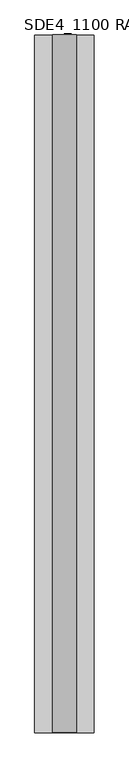
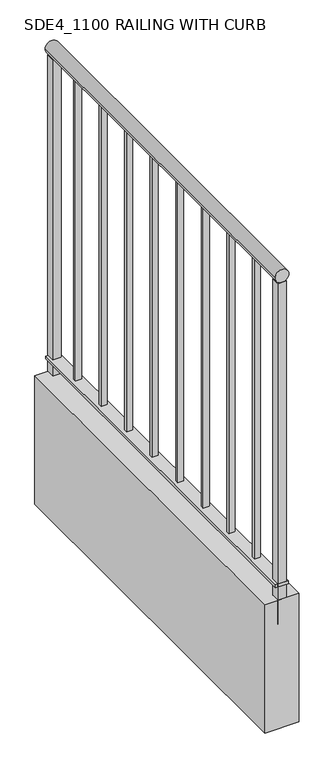
"""IFC4 building model written with IfcOpenShell, lengths in millimetres: railing geometry, SDE4_1100 RAILING WITH CURB."""

import ifcopenshell
import ifcopenshell.guid

model = None  # the IFC model being written
_history = None  # IfcOwnerHistory: only IFC2X3 demands one
_inside = {}  # id of a spatial element -> (the spatial element, [elements in it])
_under = {}  # id of a project, library or spatial element -> (it, [spatial elements below it])
_declared = {}  # id of a project -> (the project, [libraries it declares])
_typed = {}  # id of a type object -> (the type object, [elements of that type])
_made_of = {}  # id of a material, layer set ... -> (it, [elements and type objects made of it])


def new_model(schema):
    """Start an empty IFC model of exactly this schema.

    Asked for "IFC4X3", IfcOpenShell would pick the latest addendum, in which some entities
    have other attributes; the version numbers below select the first issue.
    IFC2X3 requires an IfcOwnerHistory on every rooted entity: one is made here for all.
    """
    global model, _history
    if schema == "IFC4X3":
        model = ifcopenshell.file(schema_version=(4, 3, 0, 0))
    else:
        model = ifcopenshell.file(schema=schema)
    _inside.clear()
    _under.clear()
    _declared.clear()
    _typed.clear()
    _made_of.clear()
    _history = None
    if model.schema == "IFC2X3":
        org = make("IfcOrganization", Name="unknown")
        user = make(
            "IfcPersonAndOrganization",
            ThePerson=make("IfcPerson", FamilyName="unknown"),
            TheOrganization=org,
        )
        app = make(
            "IfcApplication",
            ApplicationDeveloper=org,
            Version="unknown",
            ApplicationFullName="unknown",
            ApplicationIdentifier="unknown",
        )
        _history = make(
            "IfcOwnerHistory",
            OwningUser=user,
            OwningApplication=app,
            ChangeAction="ADDED",
            CreationDate=0,
        )
    return model


def make(cls, **values):
    """One entity of the class cls with the attributes given. An attribute that is None is left unset."""
    return model.create_entity(
        cls, **{name: value for name, value in values.items() if value is not None}
    )


def rooted(cls, **values):
    """An entity with a GlobalId (a new one), such as an element, a storey or a relation."""
    return make(cls, GlobalId=ifcopenshell.guid.new(), OwnerHistory=_history, **values)


def si_unit(unit_type, name, prefix=None):
    """IfcSIUnit, for example si_unit("LENGTHUNIT", "METRE", prefix="MILLI")."""
    return make("IfcSIUnit", UnitType=unit_type, Prefix=prefix, Name=name)


def assignment(units):
    """IfcUnitAssignment: the units of a project."""
    return None if units is None else make("IfcUnitAssignment", Units=units)


def point(xyz):
    """IfcCartesianPoint."""
    return None if xyz is None else make("IfcCartesianPoint", Coordinates=xyz)


def direction(xyz):
    """IfcDirection."""
    return None if xyz is None else make("IfcDirection", DirectionRatios=xyz)


def frame(location, z_axis=None, x_axis=None):
    """IfcAxis2Placement3D, a coordinate frame: its origin and axes. An axis left out is left unset."""
    return make(
        "IfcAxis2Placement3D",
        Location=point(location),
        Axis=direction(z_axis),
        RefDirection=direction(x_axis),
    )


def frame_2d(location, x_axis=None):
    """IfcAxis2Placement2D, a coordinate frame in the plane: its origin and x axis."""
    return make(
        "IfcAxis2Placement2D", Location=point(location), RefDirection=direction(x_axis)
    )


def origin():
    """The frame at (0, 0, 0) with its axes left unset."""
    return frame((0.0, 0.0, 0.0))


def place(relative_to, where):
    """IfcLocalPlacement: puts the frame where relative to a parent placement (None: the world)."""
    return make(
        "IfcLocalPlacement", PlacementRelTo=relative_to, RelativePlacement=where
    )


def context(
    kind, dimensions, precision=None, world=None, true_north=None, identifier=None
):
    """IfcGeometricRepresentationContext, for example the 3D "Model" context."""
    return make(
        "IfcGeometricRepresentationContext",
        ContextIdentifier=identifier,
        ContextType=kind,
        CoordinateSpaceDimension=dimensions,
        Precision=precision,
        WorldCoordinateSystem=world,
        TrueNorth=true_north,
    )


def project(units=None, contexts=None):
    """IfcProject with its units and contexts."""
    return rooted(
        "IfcProject",
        Name="project",
        RepresentationContexts=contexts,
        UnitsInContext=assignment(units),
    )


def spatial(cls, under=None, at=None, **own):
    """A site, building, storey or space (cls), placed at a placement, below another one or the project."""
    s = rooted(cls, ObjectPlacement=at, **own)
    if under is not None:
        _under.setdefault(under.id(), (under, []))[1].append(s)
    return s


def polyline(points):
    """IfcPolyline through the points."""
    return make("IfcPolyline", Points=[point(p) for p in points])


def circle_curve(where, radius):
    """IfcCircle in the frame where."""
    return make("IfcCircle", Position=where, Radius=radius)


def trimmed(basis, trim1, trim2, sense, master):
    """IfcTrimmedCurve: the piece of a basis curve between two trims."""
    return make(
        "IfcTrimmedCurve",
        BasisCurve=basis,
        Trim1=trim1,
        Trim2=trim2,
        SenseAgreement=sense,
        MasterRepresentation=master,
    )


def segment(curve, same_sense, transition):
    """IfcCompositeCurveSegment."""
    return make(
        "IfcCompositeCurveSegment",
        Transition=transition,
        SameSense=same_sense,
        ParentCurve=curve,
    )


def composite_curve(segments, self_intersect=None):
    """IfcCompositeCurve: segments joined end to end."""
    return make("IfcCompositeCurve", Segments=segments, SelfIntersect=self_intersect)


def outline(outer, holes=None, kind="AREA"):
    """IfcArbitraryClosedProfileDef: a profile drawn as a closed curve; with holes, ...WithVoids."""
    if holes is None:
        return make("IfcArbitraryClosedProfileDef", ProfileType=kind, OuterCurve=outer)
    return make(
        "IfcArbitraryProfileDefWithVoids",
        ProfileType=kind,
        OuterCurve=outer,
        InnerCurves=holes,
    )


def extrude(swept, where, along, depth):
    """IfcExtrudedAreaSolid: the profile swept, set in the frame where, extruded along a direction by depth."""
    return make(
        "IfcExtrudedAreaSolid",
        SweptArea=swept,
        Position=where,
        ExtrudedDirection=direction(along),
        Depth=depth,
    )


def shape(context_of_items, identifier, shape_type, items):
    """IfcShapeRepresentation: the items that make up one representation, for example the "Body"."""
    return make(
        "IfcShapeRepresentation",
        ContextOfItems=context_of_items,
        RepresentationIdentifier=identifier,
        RepresentationType=shape_type,
        Items=items,
    )


def source(mapping_origin, context_of_items, identifier, shape_type, items):
    """IfcRepresentationMap: a shape defined once, which mapped items show again and again."""
    return make(
        "IfcRepresentationMap",
        MappingOrigin=mapping_origin,
        MappedRepresentation=shape(context_of_items, identifier, shape_type, items),
    )


def transform(
    local_origin,
    x_axis=None,
    y_axis=None,
    z_axis=None,
    scale=None,
    scale2=None,
    scale3=None,
    uniform=True,
):
    """IfcCartesianTransformationOperator3D, or its non-uniform kind. x_axis, y_axis, z_axis: its Axis1, 2, 3."""
    if uniform:
        return make(
            "IfcCartesianTransformationOperator3D",
            Axis1=direction(x_axis),
            Axis2=direction(y_axis),
            LocalOrigin=point(local_origin),
            Scale=scale,
            Axis3=direction(z_axis),
        )
    return make(
        "IfcCartesianTransformationOperator3DnonUniform",
        Axis1=direction(x_axis),
        Axis2=direction(y_axis),
        LocalOrigin=point(local_origin),
        Scale=scale,
        Axis3=direction(z_axis),
        Scale2=scale2,
        Scale3=scale3,
    )


def mapped(mapping_source, mapping_target):
    """IfcMappedItem: shows the shape of a source again, moved by a transform."""
    return make(
        "IfcMappedItem", MappingSource=mapping_source, MappingTarget=mapping_target
    )


def made_of(thing, what):
    """Note that an element or type object is made of a material, layer set ...; save() writes the relation."""
    if what is not None:
        _made_of.setdefault(what.id(), (what, []))[1].append(thing)
    return thing


def element(
    cls,
    number,
    at=None,
    inside=None,
    cuts=None,
    type_object=None,
    material=None,
    context=None,
    identifier="Body",
    shape_type=None,
    held_by="IfcProductDefinitionShape",
    body=None,
    shapes=None,
    **own,
):
    """One element of the class cls, such as IfcWall. Its Tag is "e" and its number.

    at: its placement. inside: the storey or other place that contains it. cuts: it is an
    opening in that element (IfcRelVoidsElement). A single representation is given by context,
    identifier, shape_type and body (its items); several are given by shapes. held_by: the class
    of the entity that holds the representations. save() writes the other relations.
    """
    e = rooted(cls, Tag="e%d" % number, ObjectPlacement=at, **own)
    if body is not None:
        shapes = [shape(context, identifier, shape_type, body)]
    if shapes is not None:
        e.Representation = make(held_by, Representations=shapes)
    if inside is not None:
        _inside.setdefault(inside.id(), (inside, []))[1].append(e)
    if cuts is not None:
        rooted(
            "IfcRelVoidsElement", RelatingBuildingElement=cuts, RelatedOpeningElement=e
        )
    if type_object is not None:
        _typed.setdefault(type_object.id(), (type_object, []))[1].append(e)
    return made_of(e, material)


def aggregate(whole, parts):
    """IfcRelAggregates: a whole, such as a stair, and the parts it consists of."""
    return rooted("IfcRelAggregates", RelatingObject=whole, RelatedObjects=parts)


def save(model, path):
    """Write the relations noted so far, then the file.

    IfcRelAggregates (storeys below a building ...), IfcRelContainedInSpatialStructure (elements
    in a storey), IfcRelDefinesByType, IfcRelAssociatesMaterial and IfcRelDeclares: one each for
    every whole, place, type object, material and project.
    """
    for whole, parts in _under.values():
        aggregate(whole, parts)
    for where, things in _inside.values():
        rooted(
            "IfcRelContainedInSpatialStructure",
            RelatedElements=things,
            RelatingStructure=where,
        )
    for kind, things in _typed.values():
        rooted("IfcRelDefinesByType", RelatedObjects=things, RelatingType=kind)
    for what, things in _made_of.values():
        rooted("IfcRelAssociatesMaterial", RelatedObjects=things, RelatingMaterial=what)
    for by, libraries in _declared.values():
        rooted("IfcRelDeclares", RelatingContext=by, RelatedDefinitions=libraries)
    model.write(path)


def sde4_1100_railing_with_curb_01aa2083(model_context):
    return source(origin(), model_context, "Body", "SweptSolid", [
        extrude(outline(composite_curve([segment(trimmed(circle_curve(frame_2d((131550.0, 76500.4)), 20.0), [point((131550.0, 76520.4))], [point((131550.0, 76480.4))], False, "CARTESIAN"), True, "CONTINUOUS"), segment(trimmed(circle_curve(frame_2d((131550.0, 76500.4)), 20.0), [point((131550.0, 76480.4))], [point((131550.0, 76520.4))], False, "CARTESIAN"), True, "CONTINUOUS")], self_intersect=False)), frame((0.0, 20915.0, 0.0), z_axis=(0.0, 1.0, 0.0), x_axis=(0.0, 0.0, 1.0)), (0.0, 0.0, 1.0), 1174.1666667),
        extrude(outline(polyline([(76481.4, 22089.1666667), (76519.4, 22089.1666667), (76519.4, 20915.0), (76481.4, 20915.0), (76481.4, 22089.1666667)])), frame((0.0, 0.0, 130586.0), z_axis=(0.0, 0.0, 1.0), x_axis=(1.0, 0.0, 0.0)), (0.0, 0.0, 1.0), 9.0),
        extrude(outline(polyline([(76450.0, 22089.1666667), (76550.0, 22089.1666667), (76550.0, 20915.0), (76450.0, 20915.0), (76450.0, 22089.1666667)])), frame((0.0, 0.0, 130145.0), z_axis=(0.0, 0.0, 1.0), x_axis=(1.0, 0.0, 0.0)), (0.0, 0.0, 1.0), 400.0),
        extrude(outline(polyline([(76491.4, 21049.962963), (76509.4, 21049.962963), (76509.4, 21040.962963), (76491.4, 21040.962963), (76491.4, 21049.962963)])), frame((0.0, 0.0, 130595.0), z_axis=(0.0, 0.0, 1.0), x_axis=(1.0, 0.0, 0.0)), (0.0, 0.0, 1.0), 935.0),
        extrude(outline(polyline([(76491.4, 21180.4259259), (76509.4, 21180.4259259), (76509.4, 21171.4259259), (76491.4, 21171.4259259), (76491.4, 21180.4259259)])), frame((0.0, 0.0, 130595.0), z_axis=(0.0, 0.0, 1.0), x_axis=(1.0, 0.0, 0.0)), (0.0, 0.0, 1.0), 935.0),
        extrude(outline(polyline([(76491.4, 21310.8888889), (76509.4, 21310.8888889), (76509.4, 21301.8888889), (76491.4, 21301.8888889), (76491.4, 21310.8888889)])), frame((0.0, 0.0, 130595.0), z_axis=(0.0, 0.0, 1.0), x_axis=(1.0, 0.0, 0.0)), (0.0, 0.0, 1.0), 935.0),
        extrude(outline(polyline([(76491.4, 21441.3518519), (76509.4, 21441.3518519), (76509.4, 21432.3518519), (76491.4, 21432.3518519), (76491.4, 21441.3518519)])), frame((0.0, 0.0, 130595.0), z_axis=(0.0, 0.0, 1.0), x_axis=(1.0, 0.0, 0.0)), (0.0, 0.0, 1.0), 935.0),
        extrude(outline(polyline([(76491.4, 21571.8148148), (76509.4, 21571.8148148), (76509.4, 21562.8148148), (76491.4, 21562.8148148), (76491.4, 21571.8148148)])), frame((0.0, 0.0, 130595.0), z_axis=(0.0, 0.0, 1.0), x_axis=(1.0, 0.0, 0.0)), (0.0, 0.0, 1.0), 935.0),
        extrude(outline(polyline([(76491.4, 21702.2777778), (76509.4, 21702.2777778), (76509.4, 21693.2777778), (76491.4, 21693.2777778), (76491.4, 21702.2777778)])), frame((0.0, 0.0, 130595.0), z_axis=(0.0, 0.0, 1.0), x_axis=(1.0, 0.0, 0.0)), (0.0, 0.0, 1.0), 935.0),
        extrude(outline(polyline([(76491.4, 21832.7407407), (76509.4, 21832.7407407), (76509.4, 21823.7407407), (76491.4, 21823.7407407), (76491.4, 21832.7407407)])), frame((0.0, 0.0, 130595.0), z_axis=(0.0, 0.0, 1.0), x_axis=(1.0, 0.0, 0.0)), (0.0, 0.0, 1.0), 935.0),
        extrude(outline(polyline([(76491.4, 21963.2037037), (76509.4, 21963.2037037), (76509.4, 21954.2037037), (76491.4, 21954.2037037), (76491.4, 21963.2037037)])), frame((0.0, 0.0, 130595.0), z_axis=(0.0, 0.0, 1.0), x_axis=(1.0, 0.0, 0.0)), (0.0, 0.0, 1.0), 935.0),
        extrude(outline(polyline([(76512.9, 20940.0), (76512.9, 20915.0), (76487.9, 20915.0), (76487.9, 20940.0), (76512.9, 20940.0)])), frame((0.0, 0.0, 130470.0), z_axis=(0.0, 0.0, 1.0), x_axis=(1.0, 0.0, 0.0)), (0.0, 0.0, 1.0), 1060.0),
        extrude(outline(polyline([(76512.9, 22089.1666667), (76512.9, 22064.1666667), (76487.9, 22064.1666667), (76487.9, 22089.1666667), (76512.9, 22089.1666667)])), frame((0.0, 0.0, 130470.0), z_axis=(0.0, 0.0, 1.0), x_axis=(1.0, 0.0, 0.0)), (0.0, 0.0, 1.0), 1060.0),
    ])


if __name__ == "__main__":
    model = new_model("IFC4")
    model_context = context("Model", 3, world=origin())
    ifc_project = project(units=[si_unit("LENGTHUNIT", "METRE", prefix="MILLI")], contexts=[model_context])
    site = spatial("IfcSite", under=ifc_project)
    building = spatial("IfcBuilding", under=site)
    placement = place(None, origin())
    sde4_1100_railing_with_curb_shape = sde4_1100_railing_with_curb_01aa2083(model_context)
    element("IfcRailing", 1, ObjectType="SDE4_1100 RAILING WITH CURB", at=placement, inside=building, context=model_context, shape_type="MappedRepresentation", body=[
        mapped(sde4_1100_railing_with_curb_shape, transform((0.0, 0.0, 0.0), x_axis=(1.0, 0.0, 0.0), y_axis=(0.0, 1.0, 0.0), z_axis=(0.0, 0.0, 1.0))),
    ])
    save(model, "model.ifc")

# Revit data of these elements
# Element 1 (IfcRailing, "SDE4_1100 RAILING WITH CURB")
#   Materials on its faces: "Metal - Steel", "Concrete - Cast-in-Place Concrete"
# Materials
#   "Metal - Steel": class "Metal", colour RGB 247 247 247, transparency 0
#   "Concrete - Cast-in-Place Concrete": class "Concrete", colour RGB 191 178 173, transparency 0, Keynote = "E10/132", Cost = 0
